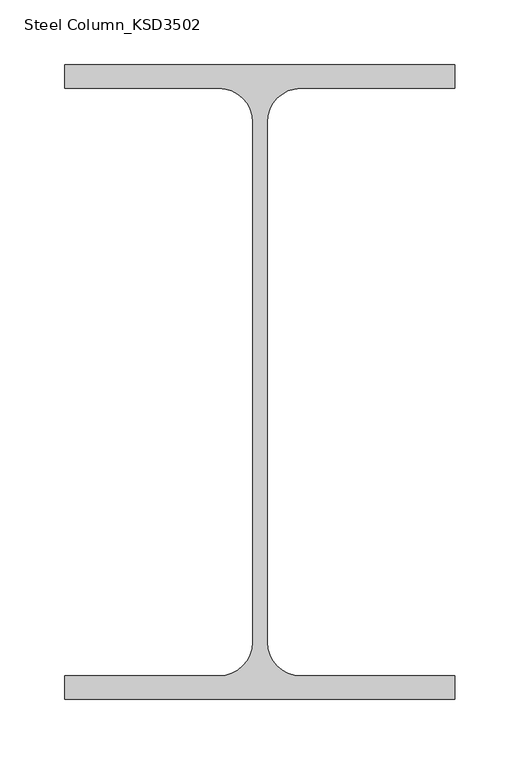
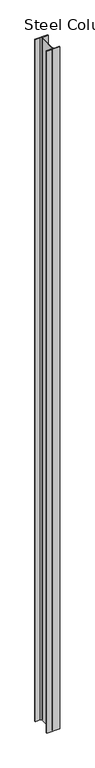
"""IFC4 building model written with IfcOpenShell, lengths in millimetres: column geometry, Steel Column_KSD3502 : H_SC_ASC_H-488×300x11x18."""

from ifc_helpers import new_model, si_unit, point, frame, frame_2d, origin, place, context, project, spatial, polyline, circle_curve, trimmed, segment, composite_curve, outline, extrude, source, transform, mapped, element, save


def steel_column_ksd3502_3ee6d03e(model_context):
    return source(origin(), model_context, "Body", "SweptSolid", [
        extrude(outline(composite_curve([segment(polyline([(150.0, 244.0), (150.0, 226.0), (31.5, 226.0)]), True, "CONTINUOUS"), segment(trimmed(circle_curve(frame_2d((31.5, 200.0)), 26.0), [point((31.5, 226.0))], [point((5.5, 200.0))], True, "CARTESIAN"), True, "CONTINUOUS"), segment(polyline([(5.5, 200.0), (5.5, -200.0)]), True, "CONTINUOUS"), segment(trimmed(circle_curve(frame_2d((31.5, -200.0)), 26.0), [point((5.5, -200.0))], [point((31.5, -226.0))], True, "CARTESIAN"), True, "CONTINUOUS"), segment(polyline([(31.5, -226.0), (150.0, -226.0), (150.0, -244.0), (-150.0, -244.0), (-150.0, -226.0), (-31.5, -226.0)]), True, "CONTINUOUS"), segment(trimmed(circle_curve(frame_2d((-31.5, -200.0)), 26.0), [point((-31.5, -226.0))], [point((-5.5, -200.0))], True, "CARTESIAN"), True, "CONTINUOUS"), segment(polyline([(-5.5, -200.0), (-5.5, 200.0)]), True, "CONTINUOUS"), segment(trimmed(circle_curve(frame_2d((-31.5, 200.0)), 26.0), [point((-5.5, 200.0))], [point((-31.5, 226.0))], True, "CARTESIAN"), True, "CONTINUOUS"), segment(polyline([(-31.5, 226.0), (-150.0, 226.0), (-150.0, 244.0), (150.0, 244.0)]), True, "CONTINUOUS")], self_intersect=False)), frame((0.0, 0.0, 685.9720055), z_axis=(0.0, 0.0, 1.0), x_axis=(1.0, 0.0, 0.0)), (0.0, 0.0, 1.0), 16914.0),
    ])


if __name__ == "__main__":
    model = new_model("IFC4")
    model_context = context("Model", 3, world=origin())
    ifc_project = project(units=[si_unit("LENGTHUNIT", "METRE", prefix="MILLI")], contexts=[model_context])
    site = spatial("IfcSite", under=ifc_project)
    building = spatial("IfcBuilding", under=site)
    placement = place(None, origin())
    steel_column_ksd3502_shape = steel_column_ksd3502_3ee6d03e(model_context)
    element("IfcColumn", 1, ObjectType="Steel Column_KSD3502 : H_SC_ASC_H-488×300x11x18", at=placement, inside=building, context=model_context, shape_type="MappedRepresentation", body=[
        mapped(steel_column_ksd3502_shape, transform((0.0, 0.0, 0.0), x_axis=(1.0, 0.0, 0.0), y_axis=(0.0, 1.0, 0.0), z_axis=(0.0, 0.0, 1.0))),
    ])
    save(model, "model.ifc")

# Revit data of these elements
# Type "Steel Column_KSD3502 : H_SC_ASC_H-488×300x11x18"
#   Width = 30.0 cm
#   Web Thickness = 1.1 cm
#   Web Fillet = 2.6 cm
#   Warping Constant = 4473230.0 cm⁶
#   Torsional Moment of Inertia = 137.492 cm⁴
#   Section Area = 163.5 cm²
#   Plastic Modulus weak axis = 830.0 cm³
#   Plastic Modulus strong axis = 3230.0 cm³
#   Perimeter = 1.27 m²/m
#   Nominal Weight = 128.00 kgf/m
#   Moment of Inertia weak axis = 8110.00 cm⁴
#   Moment of Inertia strong axis = 71000.00 cm⁴
#   Height = 48.8 cm
#   Flange Thickness = 1.8 cm
#   Elastic Modulus weak axis = 541.0 cm³
#   Elastic Modulus strong axis = 2910.0 cm³
#   Centroid Vertical = 24.4 cm
#   Centroid Horizontal = 15.0 cm
#   Bolt Spacing = 13.97 cm
#   Structural Material [instance default] = Steel, 45-345
#   Section Name Key = ""
#   Assembly Code = ""
# Element 1 (IfcColumn, "Steel Column_KSD3502 : H_SC_ASC_H-488×300x11x18")
#   Structural Material = A03AD029-00005_Anchor Bolt (Installation only)_M24
#   Materials on its faces: "A03AD029-00005_Anchor Bolt (Installation only)_M24"
# Materials
#   "Steel, 45-345": class "Metal", colour RGB 189 187 185, transparency 0, Description = "Steel 345 MPa", Cost = 0
#   "A03AD029-00005_Anchor Bolt (Installation only)_M24": class "Unassigned", colour RGB 84 83 81, transparency 0, Cost = 0
